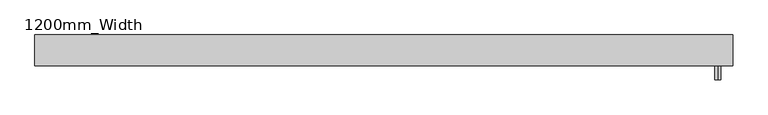
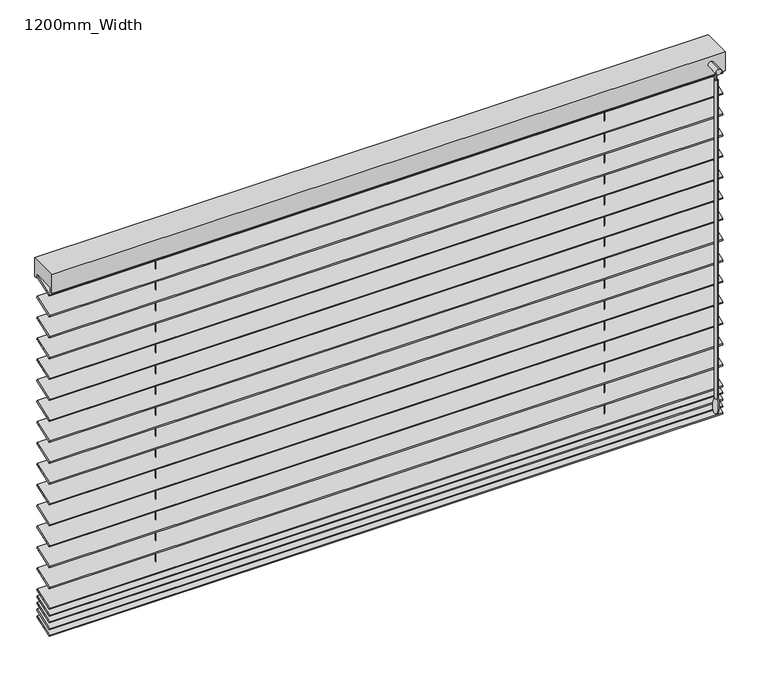
"""IFC4 building model written with IfcOpenShell, lengths in millimetres: proxy geometry, Specialty_Equipment_Venetian_Blind_Half_Down : 1200mm_Width."""

import ifcopenshell
import ifcopenshell.guid

model = None  # the IFC model being written
_history = None  # IfcOwnerHistory: only IFC2X3 demands one
_inside = {}  # id of a spatial element -> (the spatial element, [elements in it])
_under = {}  # id of a project, library or spatial element -> (it, [spatial elements below it])
_declared = {}  # id of a project -> (the project, [libraries it declares])
_typed = {}  # id of a type object -> (the type object, [elements of that type])
_made_of = {}  # id of a material, layer set ... -> (it, [elements and type objects made of it])


def new_model(schema):
    """Start an empty IFC model of exactly this schema.

    Asked for "IFC4X3", IfcOpenShell would pick the latest addendum, in which some entities
    have other attributes; the version numbers below select the first issue.
    IFC2X3 requires an IfcOwnerHistory on every rooted entity: one is made here for all.
    """
    global model, _history
    if schema == "IFC4X3":
        model = ifcopenshell.file(schema_version=(4, 3, 0, 0))
    else:
        model = ifcopenshell.file(schema=schema)
    _inside.clear()
    _under.clear()
    _declared.clear()
    _typed.clear()
    _made_of.clear()
    _history = None
    if model.schema == "IFC2X3":
        org = make("IfcOrganization", Name="unknown")
        user = make(
            "IfcPersonAndOrganization",
            ThePerson=make("IfcPerson", FamilyName="unknown"),
            TheOrganization=org,
        )
        app = make(
            "IfcApplication",
            ApplicationDeveloper=org,
            Version="unknown",
            ApplicationFullName="unknown",
            ApplicationIdentifier="unknown",
        )
        _history = make(
            "IfcOwnerHistory",
            OwningUser=user,
            OwningApplication=app,
            ChangeAction="ADDED",
            CreationDate=0,
        )
    return model


def make(cls, **values):
    """One entity of the class cls with the attributes given. An attribute that is None is left unset."""
    return model.create_entity(
        cls, **{name: value for name, value in values.items() if value is not None}
    )


def rooted(cls, **values):
    """An entity with a GlobalId (a new one), such as an element, a storey or a relation."""
    return make(cls, GlobalId=ifcopenshell.guid.new(), OwnerHistory=_history, **values)


def si_unit(unit_type, name, prefix=None):
    """IfcSIUnit, for example si_unit("LENGTHUNIT", "METRE", prefix="MILLI")."""
    return make("IfcSIUnit", UnitType=unit_type, Prefix=prefix, Name=name)


def assignment(units):
    """IfcUnitAssignment: the units of a project."""
    return None if units is None else make("IfcUnitAssignment", Units=units)


def point(xyz):
    """IfcCartesianPoint."""
    return None if xyz is None else make("IfcCartesianPoint", Coordinates=xyz)


def direction(xyz):
    """IfcDirection."""
    return None if xyz is None else make("IfcDirection", DirectionRatios=xyz)


def frame(location, z_axis=None, x_axis=None):
    """IfcAxis2Placement3D, a coordinate frame: its origin and axes. An axis left out is left unset."""
    return make(
        "IfcAxis2Placement3D",
        Location=point(location),
        Axis=direction(z_axis),
        RefDirection=direction(x_axis),
    )


def frame_2d(location, x_axis=None):
    """IfcAxis2Placement2D, a coordinate frame in the plane: its origin and x axis."""
    return make(
        "IfcAxis2Placement2D", Location=point(location), RefDirection=direction(x_axis)
    )


def origin():
    """The frame at (0, 0, 0) with its axes left unset."""
    return frame((0.0, 0.0, 0.0))


def place(relative_to, where):
    """IfcLocalPlacement: puts the frame where relative to a parent placement (None: the world)."""
    return make(
        "IfcLocalPlacement", PlacementRelTo=relative_to, RelativePlacement=where
    )


def context(
    kind, dimensions, precision=None, world=None, true_north=None, identifier=None
):
    """IfcGeometricRepresentationContext, for example the 3D "Model" context."""
    return make(
        "IfcGeometricRepresentationContext",
        ContextIdentifier=identifier,
        ContextType=kind,
        CoordinateSpaceDimension=dimensions,
        Precision=precision,
        WorldCoordinateSystem=world,
        TrueNorth=true_north,
    )


def project(units=None, contexts=None):
    """IfcProject with its units and contexts."""
    return rooted(
        "IfcProject",
        Name="project",
        RepresentationContexts=contexts,
        UnitsInContext=assignment(units),
    )


def spatial(cls, under=None, at=None, **own):
    """A site, building, storey or space (cls), placed at a placement, below another one or the project."""
    s = rooted(cls, ObjectPlacement=at, **own)
    if under is not None:
        _under.setdefault(under.id(), (under, []))[1].append(s)
    return s


def polyline(points):
    """IfcPolyline through the points."""
    return make("IfcPolyline", Points=[point(p) for p in points])


def circle_curve(where, radius):
    """IfcCircle in the frame where."""
    return make("IfcCircle", Position=where, Radius=radius)


def ellipse_curve(where, semi_axis1, semi_axis2):
    """IfcEllipse in the frame where."""
    return make(
        "IfcEllipse", Position=where, SemiAxis1=semi_axis1, SemiAxis2=semi_axis2
    )


def trimmed(basis, trim1, trim2, sense, master):
    """IfcTrimmedCurve: the piece of a basis curve between two trims."""
    return make(
        "IfcTrimmedCurve",
        BasisCurve=basis,
        Trim1=trim1,
        Trim2=trim2,
        SenseAgreement=sense,
        MasterRepresentation=master,
    )


def segment(curve, same_sense, transition):
    """IfcCompositeCurveSegment."""
    return make(
        "IfcCompositeCurveSegment",
        Transition=transition,
        SameSense=same_sense,
        ParentCurve=curve,
    )


def composite_curve(segments, self_intersect=None):
    """IfcCompositeCurve: segments joined end to end."""
    return make("IfcCompositeCurve", Segments=segments, SelfIntersect=self_intersect)


def outline(outer, holes=None, kind="AREA"):
    """IfcArbitraryClosedProfileDef: a profile drawn as a closed curve; with holes, ...WithVoids."""
    if holes is None:
        return make("IfcArbitraryClosedProfileDef", ProfileType=kind, OuterCurve=outer)
    return make(
        "IfcArbitraryProfileDefWithVoids",
        ProfileType=kind,
        OuterCurve=outer,
        InnerCurves=holes,
    )


def extrude(swept, where, along, depth):
    """IfcExtrudedAreaSolid: the profile swept, set in the frame where, extruded along a direction by depth."""
    return make(
        "IfcExtrudedAreaSolid",
        SweptArea=swept,
        Position=where,
        ExtrudedDirection=direction(along),
        Depth=depth,
    )


def shape(context_of_items, identifier, shape_type, items):
    """IfcShapeRepresentation: the items that make up one representation, for example the "Body"."""
    return make(
        "IfcShapeRepresentation",
        ContextOfItems=context_of_items,
        RepresentationIdentifier=identifier,
        RepresentationType=shape_type,
        Items=items,
    )


def source(mapping_origin, context_of_items, identifier, shape_type, items):
    """IfcRepresentationMap: a shape defined once, which mapped items show again and again."""
    return make(
        "IfcRepresentationMap",
        MappingOrigin=mapping_origin,
        MappedRepresentation=shape(context_of_items, identifier, shape_type, items),
    )


def transform(
    local_origin,
    x_axis=None,
    y_axis=None,
    z_axis=None,
    scale=None,
    scale2=None,
    scale3=None,
    uniform=True,
):
    """IfcCartesianTransformationOperator3D, or its non-uniform kind. x_axis, y_axis, z_axis: its Axis1, 2, 3."""
    if uniform:
        return make(
            "IfcCartesianTransformationOperator3D",
            Axis1=direction(x_axis),
            Axis2=direction(y_axis),
            LocalOrigin=point(local_origin),
            Scale=scale,
            Axis3=direction(z_axis),
        )
    return make(
        "IfcCartesianTransformationOperator3DnonUniform",
        Axis1=direction(x_axis),
        Axis2=direction(y_axis),
        LocalOrigin=point(local_origin),
        Scale=scale,
        Axis3=direction(z_axis),
        Scale2=scale2,
        Scale3=scale3,
    )


def mapped(mapping_source, mapping_target):
    """IfcMappedItem: shows the shape of a source again, moved by a transform."""
    return make(
        "IfcMappedItem", MappingSource=mapping_source, MappingTarget=mapping_target
    )


def made_of(thing, what):
    """Note that an element or type object is made of a material, layer set ...; save() writes the relation."""
    if what is not None:
        _made_of.setdefault(what.id(), (what, []))[1].append(thing)
    return thing


def element(
    cls,
    number,
    at=None,
    inside=None,
    cuts=None,
    type_object=None,
    material=None,
    context=None,
    identifier="Body",
    shape_type=None,
    held_by="IfcProductDefinitionShape",
    body=None,
    shapes=None,
    **own,
):
    """One element of the class cls, such as IfcWall. Its Tag is "e" and its number.

    at: its placement. inside: the storey or other place that contains it. cuts: it is an
    opening in that element (IfcRelVoidsElement). A single representation is given by context,
    identifier, shape_type and body (its items); several are given by shapes. held_by: the class
    of the entity that holds the representations. save() writes the other relations.
    """
    e = rooted(cls, Tag="e%d" % number, ObjectPlacement=at, **own)
    if body is not None:
        shapes = [shape(context, identifier, shape_type, body)]
    if shapes is not None:
        e.Representation = make(held_by, Representations=shapes)
    if inside is not None:
        _inside.setdefault(inside.id(), (inside, []))[1].append(e)
    if cuts is not None:
        rooted(
            "IfcRelVoidsElement", RelatingBuildingElement=cuts, RelatedOpeningElement=e
        )
    if type_object is not None:
        _typed.setdefault(type_object.id(), (type_object, []))[1].append(e)
    return made_of(e, material)


def aggregate(whole, parts):
    """IfcRelAggregates: a whole, such as a stair, and the parts it consists of."""
    return rooted("IfcRelAggregates", RelatingObject=whole, RelatedObjects=parts)


def save(model, path):
    """Write the relations noted so far, then the file.

    IfcRelAggregates (storeys below a building ...), IfcRelContainedInSpatialStructure (elements
    in a storey), IfcRelDefinesByType, IfcRelAssociatesMaterial and IfcRelDeclares: one each for
    every whole, place, type object, material and project.
    """
    for whole, parts in _under.values():
        aggregate(whole, parts)
    for where, things in _inside.values():
        rooted(
            "IfcRelContainedInSpatialStructure",
            RelatedElements=things,
            RelatingStructure=where,
        )
    for kind, things in _typed.values():
        rooted("IfcRelDefinesByType", RelatedObjects=things, RelatingType=kind)
    for what, things in _made_of.values():
        rooted("IfcRelAssociatesMaterial", RelatedObjects=things, RelatingMaterial=what)
    for by, libraries in _declared.values():
        rooted("IfcRelDeclares", RelatingContext=by, RelatedDefinitions=libraries)
    model.write(path)


def plane_surface(at):
    """IfcPlane: the flat surface through the origin of the frame at, square to its z axis."""
    return make("IfcPlane", Position=at)


def cylinder_surface(at, radius):
    """IfcCylindricalSurface: all points at the distance radius from the z axis of the frame at."""
    return make("IfcCylindricalSurface", Position=at, Radius=radius)


def revolved_surface(curve, axis_point, axis_direction):
    """IfcSurfaceOfRevolution: the curve turned about the line through axis_point along axis_direction."""
    return make(
        "IfcSurfaceOfRevolution",
        SweptCurve=make("IfcArbitraryOpenProfileDef", ProfileType="CURVE", Curve=curve),
        AxisPosition=make("IfcAxis1Placement", Location=point(axis_point), Axis=direction(axis_direction)),
    )


def advanced_brep(points, edges, surfaces, faces):
    """IfcAdvancedBrep: a solid bounded by faces that lie on surfaces and meet in shared edges.

    An edge is (start, end): straight between two places in points (the first is 0);
    or (start, end, curve); or (start, end, curve, False) where it runs against its curve.
    A face is (place in surfaces, loops), or (place, loops, False) where it looks against
    its surface's normal. A loop lists edges by number (the first is 1), with a minus sign
    where the edge is run from its end to its start. The first loop is the outer one.
    """
    corners = [point(p) for p in points]
    vertices = [make("IfcVertexPoint", VertexGeometry=c) for c in corners]
    made = []
    for start, end, *more in edges:
        made.append(
            make(
                "IfcEdgeCurve",
                EdgeStart=vertices[start],
                EdgeEnd=vertices[end],
                EdgeGeometry=more[0] if more else make("IfcPolyline", Points=[corners[start], corners[end]]),
                SameSense=more[1] if len(more) > 1 else True,
            )
        )
    hull = []
    for where, loops, *sense in faces:
        bounds = []
        for j, loop in enumerate(loops):
            ring = [make("IfcOrientedEdge", EdgeElement=made[abs(k) - 1], Orientation=k > 0) for k in loop]
            bounds.append(
                make(
                    "IfcFaceOuterBound" if j == 0 else "IfcFaceBound",
                    Bound=make("IfcEdgeLoop", EdgeList=ring),
                    Orientation=True,
                )
            )
        hull.append(make("IfcAdvancedFace", Bounds=bounds, FaceSurface=surfaces[where], SameSense=sense[0] if sense else True))
    return make("IfcAdvancedBrep", Outer=make("IfcClosedShell", CfsFaces=hull))


def proxy_1200mm_width_55fef7d2(model_context):
    return source(origin(), model_context, "Body", "SolidModel", [
        extrude(outline(polyline([(0.0, -40.0), (0.0, 0.0), (1180.0, 0.0), (1180.0, -40.0), (0.0, -40.0)])), frame((-439.5079376, 65.0532351, 1447.7279746), z_axis=(0.0, -0.3420201433256684, 0.9396926207859085), x_axis=(1.0, 0.0, 0.0)), (0.0, 0.0, 1.0), 3.0625345),
        extrude(outline(polyline([(0.0, -40.0), (0.0, 0.0), (1180.0, 0.0), (1180.0, -40.0), (0.0, -40.0)])), frame((-439.5079376, 65.0532351, 1459.9116214), z_axis=(0.0, -0.3420201433256684, 0.9396926207859085), x_axis=(1.0, 0.0, 0.0)), (0.0, 0.0, 1.0), 3.0625345),
        extrude(outline(polyline([(0.0, -40.0), (0.0, 0.0), (1180.0, 0.0), (1180.0, -40.0), (0.0, -40.0)])), frame((-439.5079376, 65.0532351, 1472.7202682), z_axis=(0.0, -0.3420201433256684, 0.9396926207859085), x_axis=(1.0, 0.0, 0.0)), (0.0, 0.0, 1.0), 3.0625345),
        extrude(outline(polyline([(0.0, -40.0), (0.0, 0.0), (1180.0, 0.0), (1180.0, -40.0), (0.0, -40.0)])), frame((-439.5079376, 65.0532351, 1484.903915), z_axis=(0.0, -0.3420201433256684, 0.9396926207859085), x_axis=(1.0, 0.0, 0.0)), (0.0, 0.0, 1.0), 3.0625345),
        extrude(outline(polyline([(0.0, -40.0), (0.0, 0.0), (1180.0, 0.0), (1180.0, -40.0), (0.0, -40.0)])), frame((-439.5079376, 65.0532351, 2040.2125618), z_axis=(0.0, -0.3420201433256684, 0.9396926207859085), x_axis=(1.0, 0.0, 0.0)), (0.0, 0.0, 1.0), 3.0625345),
        extrude(outline(polyline([(0.0, -40.0), (0.0, 0.0), (1180.0, 0.0), (1180.0, -40.0), (0.0, -40.0)])), frame((-439.5079376, 65.0532351, 2001.4625618), z_axis=(0.0, -0.3420201433256684, 0.9396926207859085), x_axis=(1.0, 0.0, 0.0)), (0.0, 0.0, 1.0), 3.0625345),
        extrude(outline(polyline([(0.0, -40.0), (0.0, 0.0), (1180.0, 0.0), (1180.0, -40.0), (0.0, -40.0)])), frame((-439.5079376, 65.0532351, 1962.7125618), z_axis=(0.0, -0.3420201433256684, 0.9396926207859085), x_axis=(1.0, 0.0, 0.0)), (0.0, 0.0, 1.0), 3.0625345),
        extrude(outline(polyline([(0.0, -40.0), (0.0, 0.0), (1180.0, 0.0), (1180.0, -40.0), (0.0, -40.0)])), frame((-439.5079376, 65.0532351, 1923.9625618), z_axis=(0.0, -0.3420201433256684, 0.9396926207859085), x_axis=(1.0, 0.0, 0.0)), (0.0, 0.0, 1.0), 3.0625345),
        extrude(outline(polyline([(0.0, -40.0), (0.0, 0.0), (1180.0, 0.0), (1180.0, -40.0), (0.0, -40.0)])), frame((-439.5079376, 65.0532351, 1885.2125618), z_axis=(0.0, -0.3420201433256684, 0.9396926207859085), x_axis=(1.0, 0.0, 0.0)), (0.0, 0.0, 1.0), 3.0625345),
        extrude(outline(polyline([(0.0, -40.0), (0.0, 0.0), (1180.0, 0.0), (1180.0, -40.0), (0.0, -40.0)])), frame((-439.5079376, 65.0532351, 1846.4625618), z_axis=(0.0, -0.3420201433256684, 0.9396926207859085), x_axis=(1.0, 0.0, 0.0)), (0.0, 0.0, 1.0), 3.0625345),
        extrude(outline(polyline([(0.0, -40.0), (0.0, 0.0), (1180.0, 0.0), (1180.0, -40.0), (0.0, -40.0)])), frame((-439.5079376, 65.0532351, 1807.7125618), z_axis=(0.0, -0.3420201433256684, 0.9396926207859085), x_axis=(1.0, 0.0, 0.0)), (0.0, 0.0, 1.0), 3.0625345),
        extrude(outline(polyline([(0.0, -40.0), (0.0, 0.0), (1180.0, 0.0), (1180.0, -40.0), (0.0, -40.0)])), frame((-439.5079376, 65.0532351, 1768.9625618), z_axis=(0.0, -0.3420201433256684, 0.9396926207859085), x_axis=(1.0, 0.0, 0.0)), (0.0, 0.0, 1.0), 3.0625345),
        extrude(outline(polyline([(0.0, -40.0), (0.0, 0.0), (1180.0, 0.0), (1180.0, -40.0), (0.0, -40.0)])), frame((-439.5079376, 65.0532351, 1730.2125618), z_axis=(0.0, -0.3420201433256684, 0.9396926207859085), x_axis=(1.0, 0.0, 0.0)), (0.0, 0.0, 1.0), 3.0625345),
        extrude(outline(polyline([(0.0, -40.0), (0.0, 0.0), (1180.0, 0.0), (1180.0, -40.0), (0.0, -40.0)])), frame((-439.5079376, 65.0532351, 1691.4625618), z_axis=(0.0, -0.3420201433256684, 0.9396926207859085), x_axis=(1.0, 0.0, 0.0)), (0.0, 0.0, 1.0), 3.0625345),
        extrude(outline(polyline([(0.0, -40.0), (0.0, 0.0), (1180.0, 0.0), (1180.0, -40.0), (0.0, -40.0)])), frame((-439.5079376, 65.0532351, 1652.7125618), z_axis=(0.0, -0.3420201433256684, 0.9396926207859085), x_axis=(1.0, 0.0, 0.0)), (0.0, 0.0, 1.0), 3.0625345),
        extrude(outline(polyline([(0.0, -40.0), (0.0, 0.0), (1180.0, 0.0), (1180.0, -40.0), (0.0, -40.0)])), frame((-439.5079376, 65.0532351, 1613.9625618), z_axis=(0.0, -0.3420201433256684, 0.9396926207859085), x_axis=(1.0, 0.0, 0.0)), (0.0, 0.0, 1.0), 3.0625345),
        extrude(outline(polyline([(0.0, -40.0), (0.0, 0.0), (1180.0, 0.0), (1180.0, -40.0), (0.0, -40.0)])), frame((-439.5079376, 65.0532351, 1575.2125618), z_axis=(0.0, -0.3420201433256684, 0.9396926207859085), x_axis=(1.0, 0.0, 0.0)), (0.0, 0.0, 1.0), 3.0625345),
        extrude(outline(polyline([(0.0, -40.0), (0.0, 0.0), (1180.0, 0.0), (1180.0, -40.0), (0.0, -40.0)])), frame((-439.5079376, 65.0532351, 1536.4625618), z_axis=(0.0, -0.3420201433256684, 0.9396926207859085), x_axis=(1.0, 0.0, 0.0)), (0.0, 0.0, 1.0), 3.0625345),
        extrude(outline(polyline([(0.0, -40.0), (0.0, 0.0), (1180.0, 0.0), (1180.0, -40.0), (0.0, -40.0)])), frame((-439.5079376, 65.0532351, 1497.7125618), z_axis=(0.0, -0.3420201433256684, 0.9396926207859085), x_axis=(1.0, 0.0, 0.0)), (0.0, 0.0, 1.0), 3.0625345),
        extrude(outline(polyline([(0.0, -40.0), (0.0, 0.0), (1180.0, 0.0), (1180.0, -40.0), (0.0, -40.0)])), frame((-439.5079376, 65.0532351, 2078.9625618), z_axis=(0.0, -0.3420201433256684, 0.9396926207859085), x_axis=(1.0, 0.0, 0.0)), (0.0, 0.0, 1.0), 3.0625345),
        extrude(outline(composite_curve([segment(trimmed(circle_curve(frame_2d((-242.8412709, 45.2119342)), 0.5), [point((-243.3412709, 45.2119342))], [point((-242.3412709, 45.2119342))], False, "CARTESIAN"), True, "CONTINUOUS"), segment(trimmed(circle_curve(frame_2d((-242.8412709, 45.2119342)), 0.5), [point((-242.3412709, 45.2119342))], [point((-243.3412709, 45.2119342))], False, "CARTESIAN"), True, "CONTINUOUS")], self_intersect=False)), frame((0.0, 0.0, 1434.9736305), z_axis=(0.0, 0.0, 1.0), x_axis=(1.0, 0.0, 0.0)), (0.0, 0.0, 1.0), 648.2712578),
        extrude(outline(composite_curve([segment(trimmed(circle_curve(frame_2d((543.8253958, 45.2119342)), 0.5), [point((543.3253958, 45.2119342))], [point((544.3253958, 45.2119342))], False, "CARTESIAN"), True, "CONTINUOUS"), segment(trimmed(circle_curve(frame_2d((543.8253958, 45.2119342)), 0.5), [point((544.3253958, 45.2119342))], [point((543.3253958, 45.2119342))], False, "CARTESIAN"), True, "CONTINUOUS")], self_intersect=False)), frame((0.0, 0.0, 1434.9736305), z_axis=(0.0, 0.0, 1.0), x_axis=(1.0, 0.0, 0.0)), (0.0, 0.0, 1.0), 648.2712578),
        advanced_brep(
        [(715.4920624, 4.7248495, 2091.3243671), (715.4920624, 2.7248495, 2091.3243671), (715.4920624, 3.7248495, 2091.3243671), (715.4920624, 4.7248495, 2076.3243671), (715.4920624, 2.7248495, 2076.3243671), (715.4920624, 6.7248495, 2076.3243671), (715.4920624, 0.7248495, 2076.3243671), (715.4920624, 6.7248495, 1486.909931), (715.4920624, 0.7248495, 1486.909931), (715.4920624, 7.2513368, 1460.0), (715.4920624, 0.1983622, 1460.0), (715.4920624, 3.7248495, 1460.0)],
        [
            (0, 1, circle_curve(frame((715.4920624, 3.7248495, 2091.3243671), z_axis=(0.0, 0.0, 1.0), x_axis=(0.0, -1.0, 0.0)), 1.0)),
            (1, 2),
            (2, 0),
            (1, 0, circle_curve(frame((715.4920624, 3.7248495, 2091.3243671), z_axis=(0.0, 0.0, 1.0), x_axis=(0.0, -1.0, 0.0)), 1.0)),
            (3, 4, circle_curve(frame((715.4920624, 3.7248495, 2076.3243671), z_axis=(0.0, 0.0, 1.0), x_axis=(0.0, -1.0, 0.0)), 1.0)),
            (4, 1),
            (0, 3),
            (4, 3, circle_curve(frame((715.4920624, 3.7248495, 2076.3243671), z_axis=(0.0, 0.0, 1.0), x_axis=(0.0, -1.0, 0.0)), 1.0)),
            (5, 6, circle_curve(frame((715.4920624, 3.7248495, 2076.3243671), z_axis=(0.0, 0.0, 1.0), x_axis=(0.0, -1.0, 0.0)), 3.0)),
            (6, 4),
            (3, 5),
            (6, 5, circle_curve(frame((715.4920624, 3.7248495, 2076.3243671), z_axis=(0.0, 0.0, 1.0), x_axis=(0.0, -1.0, 0.0)), 3.0)),
            (7, 8, circle_curve(frame((715.4920624, 3.7248495, 1486.909931), z_axis=(0.0, 0.0, 1.0), x_axis=(0.0, -1.0, 0.0)), 3.0)),
            (8, 6),
            (5, 7),
            (8, 7, circle_curve(frame((715.4920624, 3.7248495, 1486.909931), z_axis=(0.0, 0.0, 1.0), x_axis=(0.0, -1.0, 0.0)), 3.0)),
            (9, 10, circle_curve(frame((715.4920624, 3.7248495, 1460.0), z_axis=(0.0, 0.0, 1.0), x_axis=(0.0, -1.0, 0.0)), 3.5264873)),
            (10, 8, circle_curve(frame((715.4920624, 49.2720063, 1472.5), z_axis=(-1.0, 0.0, 0.0), x_axis=(0.0, 1.0, 0.0)), 50.6406214)),
            (7, 9, circle_curve(frame((715.4920624, -41.8223072, 1472.5), z_axis=(-1.0, 0.0, 0.0), x_axis=(0.0, -1.0, 0.0)), 50.6406214)),
            (10, 9, circle_curve(frame((715.4920624, 3.7248495, 1460.0), z_axis=(0.0, 0.0, 1.0), x_axis=(0.0, -1.0, 0.0)), 3.5264873)),
            (11, 10),
            (9, 11),
        ],
        [
            plane_surface(frame((715.4920624, 3.7248495, 2091.3243671), z_axis=(0.0, 0.0, 1.0), x_axis=(0.0, -1.0, 0.0))),
            cylinder_surface(frame((715.4920624, 3.7248495, 1191.3243671), z_axis=(0.0, 0.0, -1.0), x_axis=(0.0, -1.0, 0.0)), 1.0),
            plane_surface(frame((715.4920624, 3.7248495, 2076.3243671), z_axis=(0.0, 0.0, 1.0), x_axis=(0.0, -1.0, 0.0))),
            cylinder_surface(frame((715.4920624, 3.7248495, 1191.3243671), z_axis=(0.0, 0.0, -1.0), x_axis=(0.0, -1.0, 0.0)), 3.0),
            revolved_surface(trimmed(ellipse_curve(frame((715.4920624, 49.2720063, 1472.5), z_axis=(1.0, 0.0, 0.0), x_axis=(0.0, 1.0, 0.0)), 50.6406214, 50.6406214), [point((715.4920624, 0.7248495, 1486.909931))], [point((715.4920624, 0.1983622, 1460.0))], True, "CARTESIAN"), (715.4920624, 3.7248495, 1191.3243671), (0.0, 0.0, -1.0)),
            plane_surface(frame((715.4920624, 3.7248495, 1460.0), z_axis=(0.0, 0.0, -1.0), x_axis=(0.0, -1.0, 0.0))),
        ],
        [
            (0, [[1, 2, 3]]),
            (0, [[4, -3, -2]]),
            (1, [[5, 6, -1, 7]]),
            (1, [[8, -7, -4, -6]]),
            (2, [[9, 10, -5, 11]]),
            (2, [[12, -11, -8, -10]]),
            (3, [[13, 14, -9, 15]]),
            (3, [[16, -15, -12, -14]]),
            (4, [[17, 18, -13, 19]]),
            (4, [[20, -19, -16, -18]]),
            (5, [[21, -17, 22]]),
            (5, [[-22, -20, -21]]),
        ],
    ),
        extrude(outline(composite_curve([segment(trimmed(circle_curve(frame_2d((2095.9171213, 715.4920624)), 5.0), [point((2100.9171213, 715.4920624))], [point((2090.9171213, 715.4920624))], False, "CARTESIAN"), True, "CONTINUOUS"), segment(trimmed(circle_curve(frame_2d((2095.9171213, 715.4920624)), 5.0), [point((2090.9171213, 715.4920624))], [point((2100.9171213, 715.4920624))], False, "CARTESIAN"), True, "CONTINUOUS")], self_intersect=False)), frame((0.0, -4.4512463, 0.0), z_axis=(0.0, 1.0, 0.0), x_axis=(0.0, 0.0, 1.0)), (0.0, 0.0, 1.0), 23.7809602),
        extrude(outline(polyline([(19.329714, 2110.0), (71.0941545, 2110.0), (71.0941545, 2075.0), (66.0941545, 2075.0), (66.0941545, 2083.2448883), (24.329714, 2083.2448883), (24.329714, 2075.0), (19.329714, 2075.0), (19.329714, 2110.0)])), frame((-439.5079376, 0.0, 0.0), z_axis=(1.0, 0.0, 0.0), x_axis=(0.0, 1.0, 0.0)), (0.0, 0.0, 1.0), 1180.0),
    ])


if __name__ == "__main__":
    model = new_model("IFC4")
    model_context = context("Model", 3, world=origin())
    ifc_project = project(units=[si_unit("LENGTHUNIT", "METRE", prefix="MILLI")], contexts=[model_context])
    site = spatial("IfcSite", under=ifc_project)
    building = spatial("IfcBuilding", under=site)
    placement = place(None, origin())
    proxy_1200mm_width_shape = proxy_1200mm_width_55fef7d2(model_context)
    element("IfcBuildingElementProxy", 1, Name="Specialty_Equipment_Venetian_Blind_Half_Down : 1200mm_Width", ObjectType="Specialty_Equipment_Venetian_Blind_Half_Down : 1200mm_Width", at=placement, inside=building, context=model_context, shape_type="MappedRepresentation", body=[
        mapped(proxy_1200mm_width_shape, transform((0.0, 0.0, 0.0), x_axis=(1.0, 0.0, 0.0), y_axis=(0.0, 1.0, 0.0), z_axis=(0.0, 0.0, 1.0))),
    ])
    save(model, "model.ifc")

# Revit data of these elements
# Type "Specialty_Equipment_Venetian_Blind_Half_Down : 1200mm_Width"
#   Keynote = "N10/240"
#   Opening Width = 1200 mm
#   End Offset = 10 mm
#   Blind Length = 1180 mm
#   Blind Fixing Height = 2110 mm
#   Blind Depth = 980 mm
#   Blind Angle = 20.00°
#   Blade Depth = 40 mm
#   No of Blades = 25
#   Material Blind = Wood - Birch
# Element 1 (IfcBuildingElementProxy, "Specialty_Equipment_Venetian_Blind_Half_Down : 1200mm_Width")
#   Materials on its faces: "Wood - Birch"
# Materials
#   "Wood - Birch": class "Wood", colour RGB 224 178 126, transparency 0
